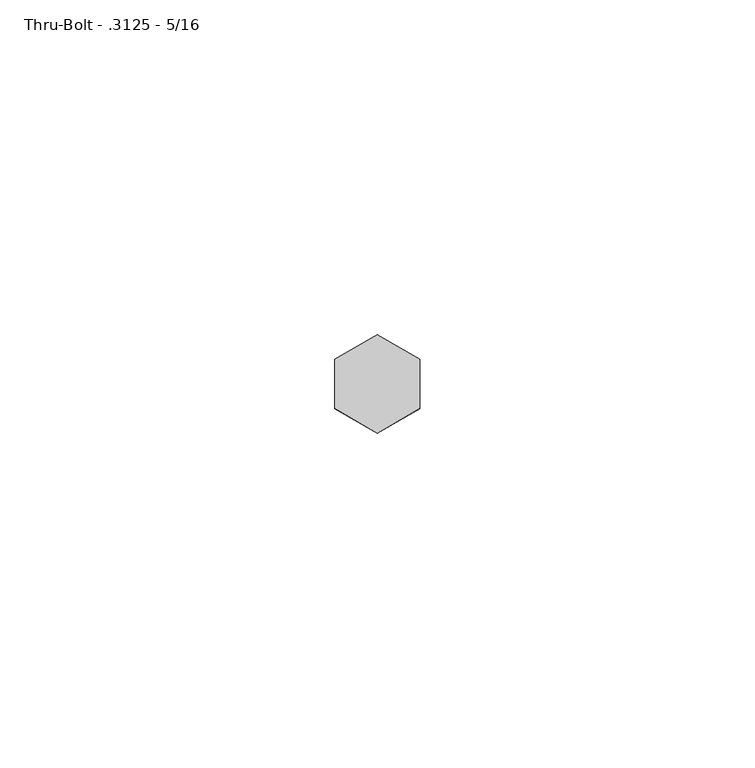
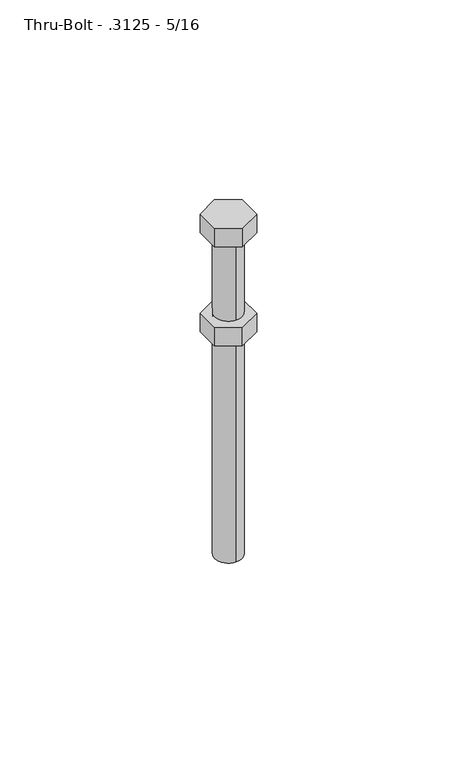
"""IFC4 building model written with IfcOpenShell, lengths in millimetres: fastener geometry, 060523 - W_P_C - Fastenings - Generic : Thru-Bolt - .3125 - 5/16."""

from ifc_helpers import new_model, si_unit, point, frame, origin, origin_with_axes, origin_2d, place, context, project, spatial, polyline, circle_curve, trimmed, segment, composite_curve, outline, extrude, source, transform, mapped, element, save


def thru_bolt_3125_5_16_482d1128(model_context):
    return source(origin(), model_context, "Body", "SweptSolid", [
        extrude(outline(polyline([(-6.35, -3.6661742), (-6.35, 3.6661742), (0.0, 7.3323484), (6.35, 3.6661742), (6.35, -3.6661742), (0.0, -7.3323484), (-6.35, -3.6661742)])), frame((0.0, 0.0, -31.353125), z_axis=(0.0, 0.0, 1.0), x_axis=(1.0, 0.0, 0.0)), (0.0, 0.0, 1.0), 5.953125),
        extrude(outline(polyline([(-6.35, 3.6661742), (0.0, 7.3323484), (6.35, 3.6661742), (6.35, -3.6661742), (0.0, -7.3323484), (-6.35, -3.6661742), (-6.35, 3.6661742)])), origin_with_axes(), (0.0, 0.0, 1.0), 5.953125),
        extrude(outline(composite_curve([segment(trimmed(circle_curve(origin_2d(), 4.1148), [point((0.0, -4.1148))], [point((0.0, 4.1148))], False, "CARTESIAN"), True, "CONTINUOUS"), segment(trimmed(circle_curve(origin_2d(), 4.1148), [point((0.0, 4.1148))], [point((0.0, -4.1148))], False, "CARTESIAN"), True, "CONTINUOUS")], self_intersect=False)), frame((0.0, 0.0, -101.6), z_axis=(0.0, 0.0, 1.0), x_axis=(1.0, 0.0, 0.0)), (0.0, 0.0, 1.0), 101.6),
    ])


if __name__ == "__main__":
    model = new_model("IFC4")
    model_context = context("Model", 3, world=origin())
    ifc_project = project(units=[si_unit("LENGTHUNIT", "METRE", prefix="MILLI")], contexts=[model_context])
    site = spatial("IfcSite", under=ifc_project)
    building = spatial("IfcBuilding", under=site)
    placement = place(None, origin())
    thru_bolt_3125_5_16_shape = thru_bolt_3125_5_16_482d1128(model_context)
    element("IfcFastener", 1, ObjectType="060523 - W_P_C - Fastenings - Generic : Thru-Bolt - .3125 - 5/16", at=placement, inside=building, context=model_context, shape_type="MappedRepresentation", body=[
        mapped(thru_bolt_3125_5_16_shape, transform((0.0, 0.0, 0.0), x_axis=(1.0, 0.0, 0.0), y_axis=(0.0, 1.0, 0.0), z_axis=(0.0, 0.0, 1.0))),
    ])
    save(model, "model.ifc")

# Revit data of these elements
# Type "060523 - W_P_C - Fastenings - Generic : Thru-Bolt - .3125 - 5/16"
#   Washer_Thickness = 0' - 0 5/64"
#   Washer Radius = 0' - 0.39638"
#   Washer Offset - Head = 0' - 0"
#   Washer Offset = 0' - 0"
#   Thickness_of_Substrate [instance default] = 0' - 1"
#   Side = 0' - 0 37/128"
#   Radius = 0' - 0.162"
#   Length [instance default] = 0' - 4"
#   Head Size = 0' - 0 1/2"
#   Head Radius = 0' - 0 1/4"
#   Head Height = 0' - 0 15/64"
#   Double Diameter = 0' - 0.648"
#   Diameter = 0' - 0.324"
#   Default Elevation = 4' - 0"
#   Washer_Nut_Visibility = no
#   Washer_Head_Visibility = no
#   Round_Head_Visibility = no
#   Point Visibility = no
#   Nut_Visibility = yes
#   Hex_Head_Visiblilty = yes
#   Washer Material = none
#   Bolt Material (Size) = AT SILL - FASTENER AT 24" O.C.
# Element 1 (IfcFastener, "060523 - W_P_C - Fastenings - Generic : Thru-Bolt - .3125 - 5/16")
#   Materials on its faces: "AT SILL - FASTENER AT 24\" O.C."
# Materials
#   "AT SILL - FASTENER AT 24\" O.C.": class "Generic", colour RGB 120 120 120, transparency 0, Cost = 0
